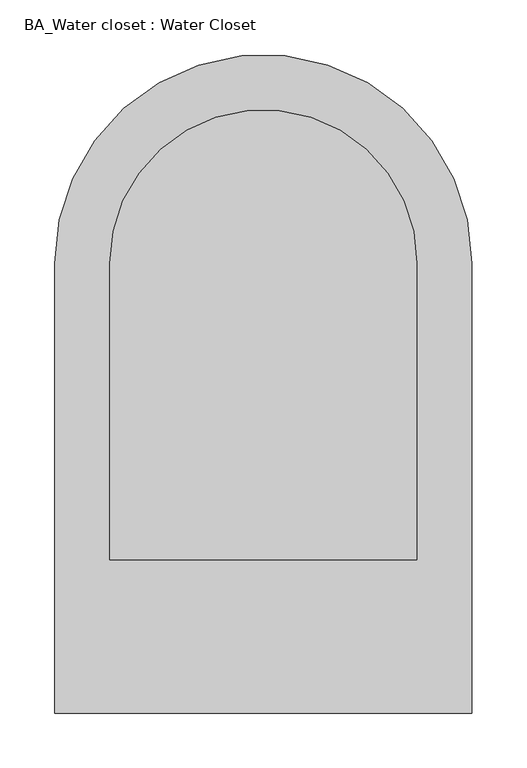
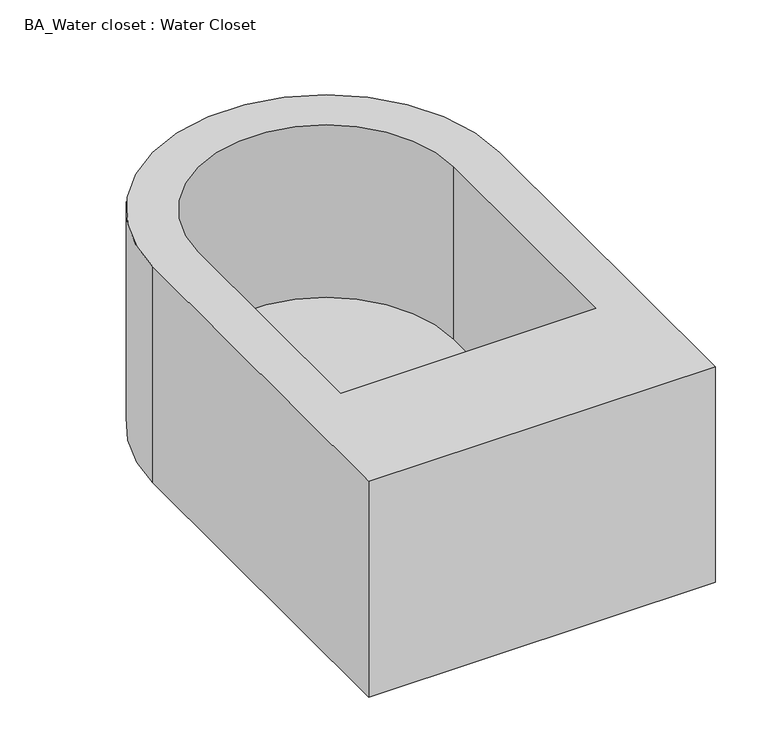
"""IFC4 building model written with IfcOpenShell, lengths in millimetres: flow terminal geometry, BA_Water closet : Water Closet."""

from ifc_helpers import new_model, si_unit, frame, origin, place, context, project, spatial, polyline, circle_curve, source, transform, mapped, element, save
from ifc_brep_helpers import plane_surface, cylinder_surface, revolved_surface, advanced_brep


def ba_water_closet_water_closet_f73c9787(model_context):
    return source(origin(), model_context, "Body", "AdvancedBrep", [
        advanced_brep(
        [(-65.0, 485.0, 400.0), (-65.0, 75.0, 400.0), (315.0, 75.0, 400.0), (315.0, 485.0, 400.0), (-15.0, 215.0, 400.0), (-15.0, 485.0, 400.0), (265.0, 485.0, 400.0), (265.0, 215.0, 400.0), (-65.0, 485.0, 150.0), (315.0, 485.0, 150.0), (315.0, 75.0, 150.0), (-65.0, 75.0, 150.0), (-15.0, 485.0, 200.0), (-15.0, 215.0, 200.0), (265.0, 215.0, 200.0), (265.0, 485.0, 200.0)],
        [
            (0, 1),
            (1, 2),
            (2, 3),
            (3, 0, circle_curve(frame((125.0, 485.0, 400.0), z_axis=(0.0, 0.0, 1.0), x_axis=(-1.0, 0.0, 0.0)), 190.0)),
            (4, 5),
            (5, 6, circle_curve(frame((125.0, 485.0, 400.0), z_axis=(0.0, 0.0, -1.0), x_axis=(-1.0, 0.0, 0.0)), 140.0)),
            (6, 7),
            (7, 4),
            (8, 9, circle_curve(frame((125.0, 485.0, 150.0), z_axis=(0.0, 0.0, -1.0), x_axis=(-1.0, 0.0, 0.0)), 190.0)),
            (9, 10),
            (10, 11),
            (11, 8),
            (0, 8),
            (11, 1),
            (10, 2),
            (9, 3),
            (12, 13),
            (13, 14),
            (14, 15),
            (15, 12, circle_curve(frame((125.0, 485.0, 200.0), z_axis=(0.0, 0.0, 1.0), x_axis=(-1.0, 0.0, 0.0)), 140.0)),
            (12, 5),
            (4, 13),
            (7, 14),
            (6, 15),
        ],
        [
            plane_surface(frame((-65.0, 75.0, 400.0), z_axis=(0.0, 0.0, 1.0), x_axis=(0.0, -1.0, 0.0))),
            plane_surface(frame((-65.0, 75.0, 150.0), z_axis=(0.0, 0.0, -1.0), x_axis=(0.0, 1.0, 0.0))),
            plane_surface(frame((-65.0, 485.0, 400.0), z_axis=(-1.0, 0.0, 0.0), x_axis=(0.0, 0.0, -1.0))),
            plane_surface(frame((-65.0, 75.0, 400.0), z_axis=(0.0, -1.0, 0.0), x_axis=(0.0, 0.0, -1.0))),
            plane_surface(frame((315.0, 75.0, 400.0), z_axis=(1.0, 0.0, 0.0), x_axis=(0.0, 0.0, -1.0))),
            plane_surface(frame((-15.0, 215.0, 200.0), z_axis=(0.0, 0.0, 1.0), x_axis=(0.0, 1.0, 0.0))),
            plane_surface(frame((-15.0, 485.0, 400.0), z_axis=(1.0, 0.0, 0.0), x_axis=(0.0, 0.0, -1.0))),
            plane_surface(frame((-15.0, 215.0, 400.0), z_axis=(0.0, 1.0, 0.0), x_axis=(0.0, 0.0, -1.0))),
            plane_surface(frame((265.0, 215.0, 400.0), z_axis=(-1.0, 0.0, 0.0), x_axis=(0.0, 0.0, -1.0))),
            cylinder_surface(frame((125.0, 485.0, 150.0), z_axis=(0.0, 0.0, 1.0), x_axis=(-1.0, 0.0, 0.0)), 190.0),
            revolved_surface(polyline([(-15.0, 485.0, 400.0), (-15.0, 485.0, 200.0)]), (125.0, 485.0, 200.0), (0.0, 0.0, 1.0)),
        ],
        [
            (0, [[1, 2, 3, 4], [5, 6, 7, 8]]),
            (1, [[9, 10, 11, 12]]),
            (2, [[-1, 13, -12, 14]]),
            (3, [[-2, -14, -11, 15]]),
            (4, [[-3, -15, -10, 16]]),
            (5, [[17, 18, 19, 20]]),
            (6, [[-17, 21, -5, 22]]),
            (7, [[-18, -22, -8, 23]]),
            (8, [[-19, -23, -7, 24]]),
            (9, [[-4, -16, -9, -13]]),
            (10, [[-20, -24, -6, -21]]),
        ],
    ),
    ])


if __name__ == "__main__":
    model = new_model("IFC4")
    model_context = context("Model", 3, world=origin())
    ifc_project = project(units=[si_unit("LENGTHUNIT", "METRE", prefix="MILLI")], contexts=[model_context])
    site = spatial("IfcSite", under=ifc_project)
    building = spatial("IfcBuilding", under=site)
    placement = place(None, origin())
    ba_water_closet_water_closet_shape = ba_water_closet_water_closet_f73c9787(model_context)
    element("IfcFlowTerminal", 1, ObjectType="BA_Water closet : Water Closet", at=placement, inside=building, context=model_context, shape_type="MappedRepresentation", body=[
        mapped(ba_water_closet_water_closet_shape, transform((0.0, 0.0, 0.0), x_axis=(1.0, 0.0, 0.0), y_axis=(0.0, 1.0, 0.0), z_axis=(0.0, 0.0, 1.0))),
    ])
    save(model, "model.ifc")

# Revit data of these elements
# Type "BA_Water closet : Water Closet"
#   height = 400 mm
#   width = 380 mm
#   depth = 600 mm
#   Default Elevation = 0
# Element 1 (IfcFlowTerminal, "BA_Water closet : Water Closet")
#   Materials on its faces: "Default"
# Materials
#   "Default": class "Generic", colour RGB 255 255 255, transparency 0, Cost = 0
